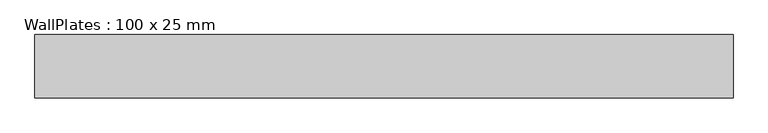
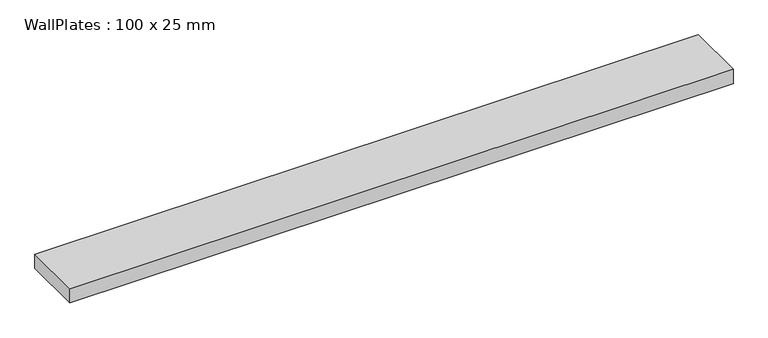
"""IFC4 building model written with IfcOpenShell, lengths in millimetres: beam geometry, WallPlates : 100 x 25 mm."""

from ifc_helpers import new_model, si_unit, frame, origin, place, context, project, spatial, polyline, outline, extrude, source, transform, mapped, element, save


def wallplates_100_x_25_mm_1ed21126(model_context):
    return source(origin(), model_context, "Body", "SweptSolid", [
        extrude(outline(polyline([(-550.0, -50.0), (-550.0, 50.0), (550.0, 50.0), (550.0, -50.0), (-550.0, -50.0)])), frame((0.0, 0.0, -12.5), z_axis=(0.0, 0.0, 1.0), x_axis=(1.0, 0.0, 0.0)), (0.0, 0.0, 1.0), 25.0),
    ])


if __name__ == "__main__":
    model = new_model("IFC4")
    model_context = context("Model", 3, world=origin())
    ifc_project = project(units=[si_unit("LENGTHUNIT", "METRE", prefix="MILLI")], contexts=[model_context])
    site = spatial("IfcSite", under=ifc_project)
    building = spatial("IfcBuilding", under=site)
    placement = place(None, origin())
    wallplates_100_x_25_mm_shape = wallplates_100_x_25_mm_1ed21126(model_context)
    element("IfcBeam", 1, ObjectType="WallPlates : 100 x 25 mm", at=placement, inside=building, context=model_context, shape_type="MappedRepresentation", body=[
        mapped(wallplates_100_x_25_mm_shape, transform((0.0, 0.0, 0.0), x_axis=(1.0, 0.0, 0.0), y_axis=(0.0, 1.0, 0.0), z_axis=(0.0, 0.0, 1.0))),
    ])
    save(model, "model.ifc")

# Revit data of these elements
# Type "WallPlates : 100 x 25 mm"
#   ExpertTruss = "Height\th\r\nWidth\tb"
#   Name [instance default] = ""
#   m [instance default] = 0 mm
#   ip_c_cut [instance default] = 1025 mm
#   h_fix [instance default] = 75 mm
#   d/2 [instance default] = 1750 mm
#   c_cut_incl [instance default] = -1000 mm
#   c_cut [instance default] = 0 mm
#   alfaMax [instance default] = 0.00°
#   alfa0_2 [instance default] = 90.00°
#   Alfa_str [instance default] = 0.00°
#   Alfa_cut [instance default] = 90.00°
#   AlfaMAX [instance default] = 0.00°
#   Alfa2_0 [instance default] = 0.00°
#   Alfa2 [instance default] = 0.00°
#   Alfa1_0 [instance default] = 0.00°
#   Alfa1 [instance default] = 0.00°
#   A_max_Str [instance default] = 0.00°
#   h_void [instance default] = 25 mm
#   beam_L_0 [instance default] = 100 mm
#   beam_L [instance default] = 0 mm
#   b_void [instance default] = 110 mm
#   alfa0_1 [instance default] = 90.00°
#   b = 100 mm
#   YOffsetStr [instance default] = 0 mm
#   YOffsetEnd [instance default] = 0 mm
#   XOffsetStr_0 [instance default] = 3500 mm
#   XOffsetStr [instance default] = 0 mm
#   XOffsetEnd_0 [instance default] = 3500 mm
#   XOffsetEnd [instance default] = 0 mm
#   L_void_0 [instance default] = 100 mm
#   L_void [instance default] = 0 mm
#   E2 [instance default] = 0.00°
#   E1 [instance default] = 0.00°
#   Length [instance default] = 3500 mm
#   h = 25 mm
#   Alfa [instance default] = 0.00°
#   A_max_End [instance default] = 0.00°
#   A_max [instance default] = 0.00°
#   A4 [instance default] = 0.00°
#   A3 [instance default] = 0.00°
#   A2 [instance default] = 0.00°
#   A1 [instance default] = 0.00°
#   Material [instance default] = Wood Standard
# Element 1 (IfcBeam, "WallPlates : 100 x 25 mm")
#   d/2 = 600 mm
#   XOffsetStr_0 = 1150 mm
#   XOffsetStr = 50 mm
#   XOffsetEnd_0 = 1150 mm
#   XOffsetEnd = 50 mm
#   Materials on its faces: "Wood Standard"
# Materials
#   "Wood Standard": class "Drewno", colour RGB 196 146 67, transparency 0, Cost = 0
